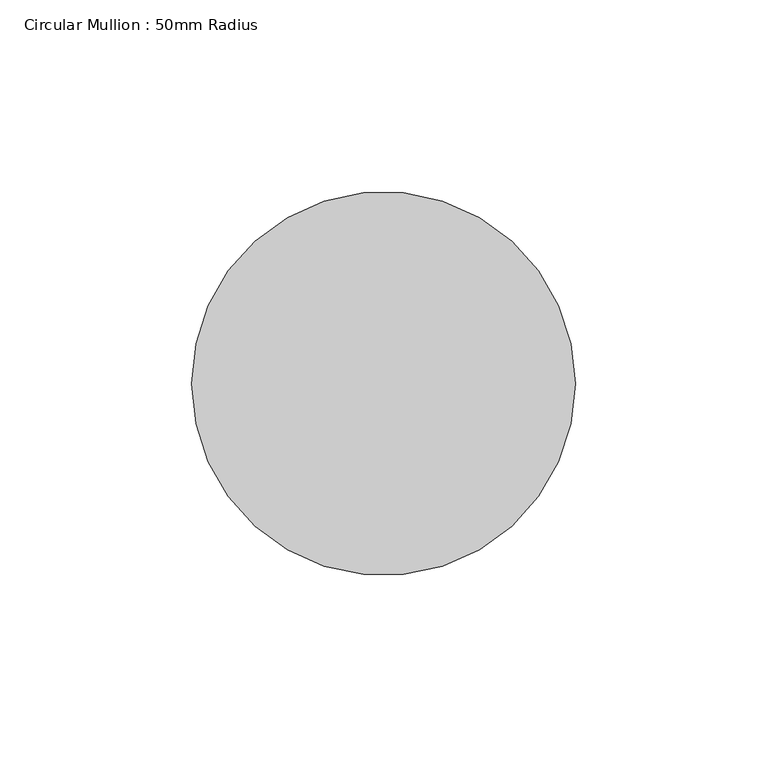
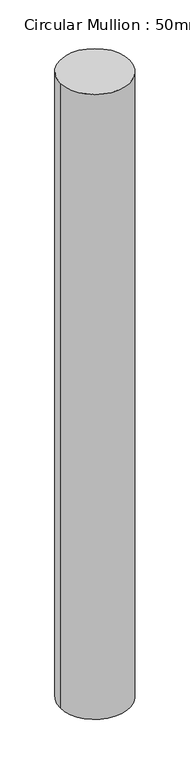
"""IFC4 building model written with IfcOpenShell, lengths in millimetres: member geometry, Circular Mullion : 50mm Radius."""

from ifc_helpers import new_model, si_unit, point, frame, origin, origin_2d, place, context, project, spatial, circle_curve, trimmed, segment, composite_curve, outline, extrude, source, transform, mapped, element, save


def circular_mullion_50mm_radius_697ab75f(model_context):
    return source(origin(), model_context, "Body", "SweptSolid", [
        extrude(outline(composite_curve([segment(trimmed(circle_curve(origin_2d(), 50.0), [point((50.0, 0.0))], [point((-50.0, 0.0))], False, "CARTESIAN"), True, "CONTINUOUS"), segment(trimmed(circle_curve(origin_2d(), 50.0), [point((-50.0, 0.0))], [point((50.0, 0.0))], False, "CARTESIAN"), True, "CONTINUOUS")], self_intersect=False)), frame((0.0, 0.0, -951.532032), z_axis=(0.0, 0.0, 1.0), x_axis=(1.0, 0.0, 0.0)), (0.0, 0.0, 1.0), 951.532032),
    ])


if __name__ == "__main__":
    model = new_model("IFC4")
    model_context = context("Model", 3, world=origin())
    ifc_project = project(units=[si_unit("LENGTHUNIT", "METRE", prefix="MILLI")], contexts=[model_context])
    site = spatial("IfcSite", under=ifc_project)
    building = spatial("IfcBuilding", under=site)
    placement = place(None, origin())
    circular_mullion_50mm_radius_shape = circular_mullion_50mm_radius_697ab75f(model_context)
    element("IfcMember", 1, ObjectType="Circular Mullion : 50mm Radius", at=placement, inside=building, context=model_context, shape_type="MappedRepresentation", body=[
        mapped(circular_mullion_50mm_radius_shape, transform((0.0, 0.0, 0.0), x_axis=(1.0, 0.0, 0.0), y_axis=(0.0, 1.0, 0.0), z_axis=(0.0, 0.0, 1.0))),
    ])
    save(model, "model.ifc")

# Revit data of these elements
# Type "Circular Mullion : 50mm Radius"
#   built-in parameter 1007350 = 0.164042 (stored number, unit not read)
# Element 1 (IfcMember, "Circular Mullion : 50mm Radius")
#   Materials on its faces: "Aluminium"
# Materials
#   "Aluminium": class "Metal", colour RGB 247 247 247, transparency 0, Description = "Aluminium 6061", Cost = 0
